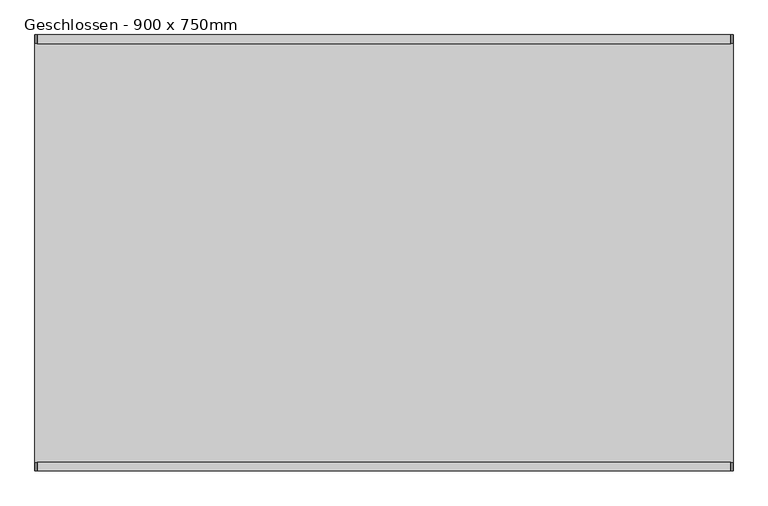
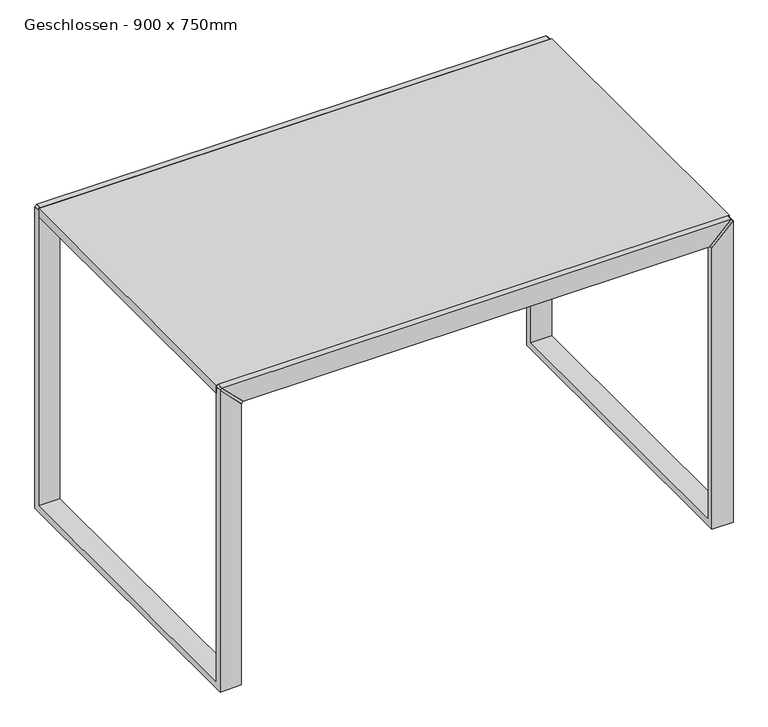
"""IFC4 building model written with IfcOpenShell, lengths in millimetres: furniture geometry, Tisch - Klassiker : Geschlossen - 900 x 750mm."""

import ifcopenshell
import ifcopenshell.guid

model = None  # the IFC model being written
_history = None  # IfcOwnerHistory: only IFC2X3 demands one
_inside = {}  # id of a spatial element -> (the spatial element, [elements in it])
_under = {}  # id of a project, library or spatial element -> (it, [spatial elements below it])
_declared = {}  # id of a project -> (the project, [libraries it declares])
_typed = {}  # id of a type object -> (the type object, [elements of that type])
_made_of = {}  # id of a material, layer set ... -> (it, [elements and type objects made of it])


def new_model(schema):
    """Start an empty IFC model of exactly this schema.

    Asked for "IFC4X3", IfcOpenShell would pick the latest addendum, in which some entities
    have other attributes; the version numbers below select the first issue.
    IFC2X3 requires an IfcOwnerHistory on every rooted entity: one is made here for all.
    """
    global model, _history
    if schema == "IFC4X3":
        model = ifcopenshell.file(schema_version=(4, 3, 0, 0))
    else:
        model = ifcopenshell.file(schema=schema)
    _inside.clear()
    _under.clear()
    _declared.clear()
    _typed.clear()
    _made_of.clear()
    _history = None
    if model.schema == "IFC2X3":
        org = make("IfcOrganization", Name="unknown")
        user = make(
            "IfcPersonAndOrganization",
            ThePerson=make("IfcPerson", FamilyName="unknown"),
            TheOrganization=org,
        )
        app = make(
            "IfcApplication",
            ApplicationDeveloper=org,
            Version="unknown",
            ApplicationFullName="unknown",
            ApplicationIdentifier="unknown",
        )
        _history = make(
            "IfcOwnerHistory",
            OwningUser=user,
            OwningApplication=app,
            ChangeAction="ADDED",
            CreationDate=0,
        )
    return model


def make(cls, **values):
    """One entity of the class cls with the attributes given. An attribute that is None is left unset."""
    return model.create_entity(
        cls, **{name: value for name, value in values.items() if value is not None}
    )


def rooted(cls, **values):
    """An entity with a GlobalId (a new one), such as an element, a storey or a relation."""
    return make(cls, GlobalId=ifcopenshell.guid.new(), OwnerHistory=_history, **values)


def si_unit(unit_type, name, prefix=None):
    """IfcSIUnit, for example si_unit("LENGTHUNIT", "METRE", prefix="MILLI")."""
    return make("IfcSIUnit", UnitType=unit_type, Prefix=prefix, Name=name)


def assignment(units):
    """IfcUnitAssignment: the units of a project."""
    return None if units is None else make("IfcUnitAssignment", Units=units)


def point(xyz):
    """IfcCartesianPoint."""
    return None if xyz is None else make("IfcCartesianPoint", Coordinates=xyz)


def direction(xyz):
    """IfcDirection."""
    return None if xyz is None else make("IfcDirection", DirectionRatios=xyz)


def frame(location, z_axis=None, x_axis=None):
    """IfcAxis2Placement3D, a coordinate frame: its origin and axes. An axis left out is left unset."""
    return make(
        "IfcAxis2Placement3D",
        Location=point(location),
        Axis=direction(z_axis),
        RefDirection=direction(x_axis),
    )


def origin():
    """The frame at (0, 0, 0) with its axes left unset."""
    return frame((0.0, 0.0, 0.0))


def place(relative_to, where):
    """IfcLocalPlacement: puts the frame where relative to a parent placement (None: the world)."""
    return make(
        "IfcLocalPlacement", PlacementRelTo=relative_to, RelativePlacement=where
    )


def context(
    kind, dimensions, precision=None, world=None, true_north=None, identifier=None
):
    """IfcGeometricRepresentationContext, for example the 3D "Model" context."""
    return make(
        "IfcGeometricRepresentationContext",
        ContextIdentifier=identifier,
        ContextType=kind,
        CoordinateSpaceDimension=dimensions,
        Precision=precision,
        WorldCoordinateSystem=world,
        TrueNorth=true_north,
    )


def project(units=None, contexts=None):
    """IfcProject with its units and contexts."""
    return rooted(
        "IfcProject",
        Name="project",
        RepresentationContexts=contexts,
        UnitsInContext=assignment(units),
    )


def spatial(cls, under=None, at=None, **own):
    """A site, building, storey or space (cls), placed at a placement, below another one or the project."""
    s = rooted(cls, ObjectPlacement=at, **own)
    if under is not None:
        _under.setdefault(under.id(), (under, []))[1].append(s)
    return s


def polyline(points):
    """IfcPolyline through the points."""
    return make("IfcPolyline", Points=[point(p) for p in points])


def outline(outer, holes=None, kind="AREA"):
    """IfcArbitraryClosedProfileDef: a profile drawn as a closed curve; with holes, ...WithVoids."""
    if holes is None:
        return make("IfcArbitraryClosedProfileDef", ProfileType=kind, OuterCurve=outer)
    return make(
        "IfcArbitraryProfileDefWithVoids",
        ProfileType=kind,
        OuterCurve=outer,
        InnerCurves=holes,
    )


def extrude(swept, where, along, depth):
    """IfcExtrudedAreaSolid: the profile swept, set in the frame where, extruded along a direction by depth."""
    return make(
        "IfcExtrudedAreaSolid",
        SweptArea=swept,
        Position=where,
        ExtrudedDirection=direction(along),
        Depth=depth,
    )


def faces_of(points, faces, orient=None, outer=None):
    """IfcFace entities. A face is a list of loops; a loop is a list of indices into points, from 0.

    orient and outer hold one flag for each loop. By default every Orientation is true, the
    first loop of a face is its IfcFaceOuterBound and the others are IfcFaceBound.
    """
    made = []
    for i, loops in enumerate(faces):
        bounds = []
        for j, loop in enumerate(loops):
            is_outer = j == 0 if outer is None else outer[i][j]
            bounds.append(
                make(
                    "IfcFaceOuterBound" if is_outer else "IfcFaceBound",
                    Bound=make("IfcPolyLoop", Polygon=[points[k] for k in loop]),
                    Orientation=True if orient is None else orient[i][j],
                )
            )
        made.append(make("IfcFace", Bounds=bounds))
    return made


def faceted_brep(points, faces, orient=None, outer=None, voids=None):
    """IfcFacetedBrep: a solid bounded by flat faces; with voids (closed shells), ...WithVoids."""
    shared = [point(p) for p in points]
    hull = make("IfcClosedShell", CfsFaces=faces_of(shared, faces, orient, outer))
    if voids is None:
        return make("IfcFacetedBrep", Outer=hull)
    return make(
        "IfcFacetedBrepWithVoids",
        Outer=hull,
        Voids=[
            make(cls, CfsFaces=faces_of(shared, fs, o, b)) for cls, fs, o, b in voids
        ],
    )


def shape(context_of_items, identifier, shape_type, items):
    """IfcShapeRepresentation: the items that make up one representation, for example the "Body"."""
    return make(
        "IfcShapeRepresentation",
        ContextOfItems=context_of_items,
        RepresentationIdentifier=identifier,
        RepresentationType=shape_type,
        Items=items,
    )


def source(mapping_origin, context_of_items, identifier, shape_type, items):
    """IfcRepresentationMap: a shape defined once, which mapped items show again and again."""
    return make(
        "IfcRepresentationMap",
        MappingOrigin=mapping_origin,
        MappedRepresentation=shape(context_of_items, identifier, shape_type, items),
    )


def transform(
    local_origin,
    x_axis=None,
    y_axis=None,
    z_axis=None,
    scale=None,
    scale2=None,
    scale3=None,
    uniform=True,
):
    """IfcCartesianTransformationOperator3D, or its non-uniform kind. x_axis, y_axis, z_axis: its Axis1, 2, 3."""
    if uniform:
        return make(
            "IfcCartesianTransformationOperator3D",
            Axis1=direction(x_axis),
            Axis2=direction(y_axis),
            LocalOrigin=point(local_origin),
            Scale=scale,
            Axis3=direction(z_axis),
        )
    return make(
        "IfcCartesianTransformationOperator3DnonUniform",
        Axis1=direction(x_axis),
        Axis2=direction(y_axis),
        LocalOrigin=point(local_origin),
        Scale=scale,
        Axis3=direction(z_axis),
        Scale2=scale2,
        Scale3=scale3,
    )


def mapped(mapping_source, mapping_target):
    """IfcMappedItem: shows the shape of a source again, moved by a transform."""
    return make(
        "IfcMappedItem", MappingSource=mapping_source, MappingTarget=mapping_target
    )


def made_of(thing, what):
    """Note that an element or type object is made of a material, layer set ...; save() writes the relation."""
    if what is not None:
        _made_of.setdefault(what.id(), (what, []))[1].append(thing)
    return thing


def element(
    cls,
    number,
    at=None,
    inside=None,
    cuts=None,
    type_object=None,
    material=None,
    context=None,
    identifier="Body",
    shape_type=None,
    held_by="IfcProductDefinitionShape",
    body=None,
    shapes=None,
    **own,
):
    """One element of the class cls, such as IfcWall. Its Tag is "e" and its number.

    at: its placement. inside: the storey or other place that contains it. cuts: it is an
    opening in that element (IfcRelVoidsElement). A single representation is given by context,
    identifier, shape_type and body (its items); several are given by shapes. held_by: the class
    of the entity that holds the representations. save() writes the other relations.
    """
    e = rooted(cls, Tag="e%d" % number, ObjectPlacement=at, **own)
    if body is not None:
        shapes = [shape(context, identifier, shape_type, body)]
    if shapes is not None:
        e.Representation = make(held_by, Representations=shapes)
    if inside is not None:
        _inside.setdefault(inside.id(), (inside, []))[1].append(e)
    if cuts is not None:
        rooted(
            "IfcRelVoidsElement", RelatingBuildingElement=cuts, RelatedOpeningElement=e
        )
    if type_object is not None:
        _typed.setdefault(type_object.id(), (type_object, []))[1].append(e)
    return made_of(e, material)


def aggregate(whole, parts):
    """IfcRelAggregates: a whole, such as a stair, and the parts it consists of."""
    return rooted("IfcRelAggregates", RelatingObject=whole, RelatedObjects=parts)


def save(model, path):
    """Write the relations noted so far, then the file.

    IfcRelAggregates (storeys below a building ...), IfcRelContainedInSpatialStructure (elements
    in a storey), IfcRelDefinesByType, IfcRelAssociatesMaterial and IfcRelDeclares: one each for
    every whole, place, type object, material and project.
    """
    for whole, parts in _under.values():
        aggregate(whole, parts)
    for where, things in _inside.values():
        rooted(
            "IfcRelContainedInSpatialStructure",
            RelatedElements=things,
            RelatingStructure=where,
        )
    for kind, things in _typed.values():
        rooted("IfcRelDefinesByType", RelatedObjects=things, RelatingType=kind)
    for what, things in _made_of.values():
        rooted("IfcRelAssociatesMaterial", RelatedObjects=things, RelatingMaterial=what)
    for by, libraries in _declared.values():
        rooted("IfcRelDeclares", RelatingContext=by, RelatedDefinitions=libraries)
    model.write(path)


def geschlossen_900_x_750mm_e7da02b5(model_context):
    return source(origin(), model_context, "Body", "SolidModel", [
        extrude(outline(polyline([(15.0, 0.0), (15.0, -70.7106781), (0.0, -70.7106781), (0.0, 0.0), (15.0, 0.0)])), frame((-600.0, -375.0, 745.7573593), z_axis=(0.7071067811865495, 0.0, 0.7071067811865456), x_axis=(0.0, 1.0, 0.0)), (0.0, 0.0, 1.0), 6.0),
        extrude(outline(polyline([(1375.8582233, 0.0), (1375.8582233, -15.0), (1305.1475452, -15.0), (1305.1475452, 0.0), (1375.8582233, 0.0)])), frame((372.8786797, 360.0, -227.1213203), z_axis=(0.7071067811865495, 0.0, 0.7071067811865456), x_axis=(-0.7071067811865456, 0.0, 0.7071067811865495)), (0.0, 0.0, 1.0), 6.0),
        extrude(outline(polyline([(0.0, -15.0), (0.0, 0.0), (6.0, 0.0), (6.0, -15.0), (0.0, -15.0)])), frame((545.7573593, 375.0, 700.0), z_axis=(0.7071067811865419, 0.0, 0.7071067811865532), x_axis=(0.7071067811865532, 0.0, -0.7071067811865419)), (0.0, 0.0, 1.0), 70.7106781),
        extrude(outline(polyline([(0.0, -15.0), (0.0, 0.0), (6.0, 0.0), (6.0, -15.0), (0.0, -15.0)])), frame((545.7573593, -360.0, 700.0), z_axis=(0.7071067811865476, 0.0, 0.7071067811865476), x_axis=(0.7071067811865476, 0.0, -0.7071067811865476)), (0.0, 0.0, 1.0), 70.7106781),
        extrude(outline(polyline([(335.0, 360.0), (350.0, 360.0), (350.0, -360.0), (335.0, -360.0), (335.0, 360.0)])), frame((0.0, 0.0, 700.0), z_axis=(0.0, 0.0, 1.0), x_axis=(1.0, 0.0, 0.0)), (0.0, 0.0, 1.0), 30.0),
        extrude(outline(polyline([(515.0, 360.0), (530.0, 360.0), (530.0, -360.0), (515.0, -360.0), (515.0, 360.0)])), frame((0.0, 0.0, 700.0), z_axis=(0.0, 0.0, 1.0), x_axis=(1.0, 0.0, 0.0)), (0.0, 0.0, 1.0), 30.0),
        faceted_brep([(550.0, -360.0, 695.7573593), (600.0, -360.0, 745.7573593), (600.0, -360.0, 15.0), (550.0, -360.0, 15.0), (600.0, -375.0, 745.7573593), (550.0, -375.0, 695.7573593), (550.0, -375.0, 0.0), (600.0, -375.0, 0.0), (600.0, 375.0, 0.0), (600.0, 375.0, 745.7573593), (600.0, 360.0, 745.7573593), (600.0, 360.0, 15.0), (550.0, 375.0, 0.0), (550.0, 360.0, 15.0), (550.0, 360.0, 695.7573593), (550.0, 375.0, 695.7573593)], [[[0, 1, 2, 3]], [[4, 5, 6, 7]], [[1, 4, 7, 8, 9, 10, 11, 2]], [[8, 7, 6, 12]], [[5, 0, 3, 13, 14, 15, 12, 6]], [[1, 0, 5, 4]], [[3, 2, 11, 13]], [[9, 8, 12, 15]], [[10, 14, 13, 11]], [[9, 15, 14, 10]]]),
        faceted_brep([(-600.0, -360.0, 745.7573593), (-550.0, -360.0, 695.7573593), (-550.0, -360.0, 15.0), (-600.0, -360.0, 15.0), (-600.0, -375.0, 0.0), (-550.0, -375.0, 0.0), (-550.0, -375.0, 695.7573593), (-600.0, -375.0, 745.7573593), (-550.0, 375.0, 0.0), (-600.0, 375.0, 0.0), (-550.0, 375.0, 695.7573593), (-550.0, 360.0, 695.7573593), (-550.0, 360.0, 15.0), (-600.0, 360.0, 15.0), (-600.0, 360.0, 745.7573593), (-600.0, 375.0, 745.7573593)], [[[0, 1, 2, 3]], [[4, 5, 6, 7]], [[8, 5, 4, 9]], [[1, 0, 7, 6]], [[1, 6, 5, 8, 10, 11, 12, 2]], [[7, 0, 3, 13, 14, 15, 9, 4]], [[3, 2, 12, 13]], [[9, 15, 10, 8]], [[11, 14, 13, 12]], [[10, 15, 14, 11]]]),
        extrude(outline(polyline([(700.0, -545.7573593), (700.0, 545.7573593), (750.0, 595.7573593), (750.0, -595.7573593), (700.0, -545.7573593)])), frame((0.0, 360.0, 0.0), z_axis=(0.0, 1.0, 0.0), x_axis=(0.0, 0.0, 1.0)), (0.0, 0.0, 1.0), 15.0),
        extrude(outline(polyline([(700.0, -545.7573593), (700.0, 545.7573593), (750.0, 595.7573593), (750.0, -595.7573593), (700.0, -545.7573593)])), frame((0.0, -375.0, 0.0), z_axis=(0.0, 1.0, 0.0), x_axis=(0.0, 0.0, 1.0)), (0.0, 0.0, 1.0), 15.0),
        extrude(outline(polyline([(600.0, 360.0), (600.0, -360.0), (-600.0, -360.0), (-600.0, 360.0), (600.0, 360.0)])), frame((0.0, 0.0, 730.0), z_axis=(0.0, 0.0, 1.0), x_axis=(1.0, 0.0, 0.0)), (0.0, 0.0, 1.0), 20.0),
    ])


if __name__ == "__main__":
    model = new_model("IFC4")
    model_context = context("Model", 3, world=origin())
    ifc_project = project(units=[si_unit("LENGTHUNIT", "METRE", prefix="MILLI")], contexts=[model_context])
    site = spatial("IfcSite", under=ifc_project)
    building = spatial("IfcBuilding", under=site)
    placement = place(None, origin())
    geschlossen_900_x_750mm_shape = geschlossen_900_x_750mm_e7da02b5(model_context)
    element("IfcFurniture", 1, ObjectType="Tisch - Klassiker : Geschlossen - 900 x 750mm", at=placement, inside=building, context=model_context, shape_type="MappedRepresentation", body=[
        mapped(geschlossen_900_x_750mm_shape, transform((0.0, 0.0, 0.0), x_axis=(1.0, 0.0, 0.0), y_axis=(0.0, 1.0, 0.0), z_axis=(0.0, 0.0, 1.0))),
    ])
    save(model, "model.ifc")

# Revit data of these elements
# Type "Tisch - Klassiker : Geschlossen - 900 x 750mm"
#   Breite = 1.200 m
#   Tischplatte = Emaille - Grau
#   Fuß = Metall - Aluminium
#   Type Comments = ""
# Element 1 (IfcFurniture, "Tisch - Klassiker : Geschlossen - 900 x 750mm")
#   Materials on its faces: "Metall - Aluminium", "Holz - Birke", "Emaille - Grau"
# Materials
#   "Emaille - Grau": class "Keramik", colour RGB 103 105 109, transparency 0
#   "Metall - Aluminium": class "Metall", colour RGB 247 247 247, transparency 0, Description = "Aluminium 6061", Cost = 0
#   "Holz - Birke": class "Holz", colour RGB 213 164 103, transparency 0, Cost = 0
